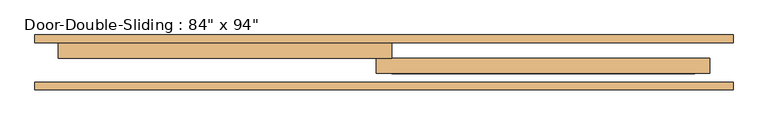
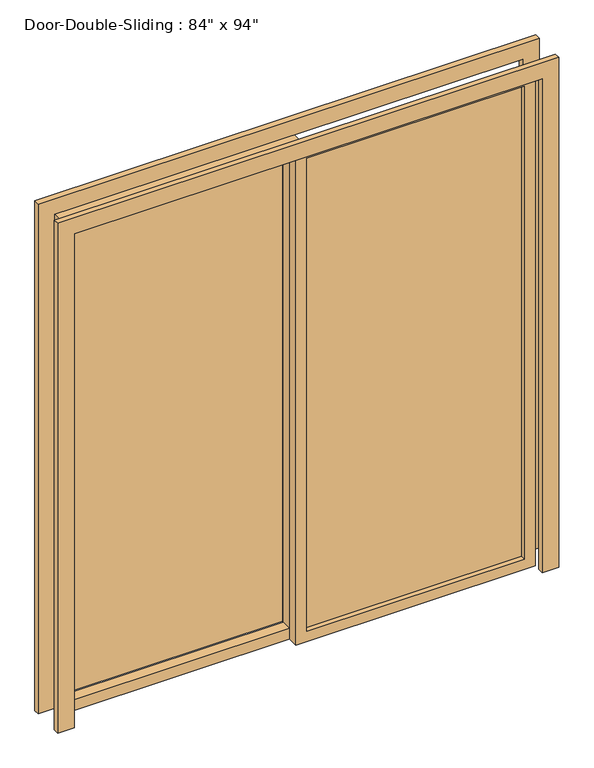
"""IFC4 building model written with IfcOpenShell, lengths in millimetres: door geometry."""

from ifc_helpers import new_model, si_unit, frame, origin, place, context, project, spatial, polyline, outline, extrude, source, transform, mapped, element, save


def door_ba072b10(model_context):
    return source(origin(), model_context, "Body", "SweptSolid", [
        extrude(outline(polyline([(0.0, 1151.2), (2476.2, 1151.2), (2476.2, -1151.2), (0.0, -1151.2), (0.0, -1075.0), (2400.0, -1075.0), (2400.0, 1075.0), (0.0, 1075.0), (0.0, 1151.2)])), frame((0.0, 192.0, 0.0), z_axis=(0.0, 1.0, 0.0), x_axis=(0.0, 0.0, 1.0)), (0.0, 0.0, 1.0), 25.4),
        extrude(outline(polyline([(0.0, -1151.2), (0.0, -1075.0), (2400.0, -1075.0), (2400.0, 1075.0), (0.0, 1075.0), (0.0, 1151.2), (2476.2, 1151.2), (2476.2, -1151.2), (0.0, -1151.2)])), frame((0.0, 36.6, 0.0), z_axis=(0.0, 1.0, 0.0), x_axis=(0.0, 0.0, 1.0)), (0.0, 0.0, 1.0), 25.4),
        extrude(outline(polyline([(2400.0, 25.4), (2400.0, -1075.0), (0.0, -1075.0), (0.0, 25.4), (2400.0, 25.4)]), holes=[polyline([(2349.2, -25.4), (50.8, -25.4), (50.8, -1024.2), (2349.2, -1024.2), (2349.2, -25.4)])]), frame((0.0, 141.2, 0.0), z_axis=(0.0, 1.0, 0.0), x_axis=(0.0, 0.0, 1.0)), (0.0, 0.0, 1.0), 50.8),
        extrude(outline(polyline([(2400.0, -25.4), (0.0, -25.4), (0.0, 1075.0), (2400.0, 1075.0), (2400.0, -25.4)]), holes=[polyline([(2349.2, 25.4), (2349.2, 1024.2), (50.8, 1024.2), (50.8, 25.4), (2349.2, 25.4)])]), frame((0.0, 90.4, 0.0), z_axis=(0.0, 1.0, 0.0), x_axis=(0.0, 0.0, 1.0)), (0.0, 0.0, 1.0), 50.8),
        extrude(outline(polyline([(-25.4, 200.025), (-1024.2, 200.025), (-1024.2, 206.375), (-25.4, 206.375), (-25.4, 200.025)])), frame((0.0, 0.0, 50.8), z_axis=(0.0, 0.0, 1.0), x_axis=(1.0, 0.0, 0.0)), (0.0, 0.0, 1.0), 2298.4),
        extrude(outline(polyline([(25.4, 118.975), (1024.2, 118.975), (1024.2, 112.625), (25.4, 112.625), (25.4, 118.975)])), frame((0.0, 0.0, 50.8), z_axis=(0.0, 0.0, 1.0), x_axis=(1.0, 0.0, 0.0)), (0.0, 0.0, 1.0), 2298.4),
    ])


if __name__ == "__main__":
    model = new_model("IFC4")
    model_context = context("Model", 3, world=origin())
    ifc_project = project(units=[si_unit("LENGTHUNIT", "METRE", prefix="MILLI")], contexts=[model_context])
    site = spatial("IfcSite", under=ifc_project)
    building = spatial("IfcBuilding", under=site)
    placement = place(None, origin())
    door_shape = door_ba072b10(model_context)
    element("IfcDoor", 1, ObjectType="Door-Double-Sliding : 84\" x 94\"", at=placement, inside=building, context=model_context, shape_type="MappedRepresentation", body=[
        mapped(door_shape, transform((0.0, 0.0, 0.0), x_axis=(1.0, 0.0, 0.0), y_axis=(0.0, 1.0, 0.0), z_axis=(0.0, 0.0, 1.0))),
    ])
    save(model, "model.ifc")

# Revit data of these elements
# Type "Door-Double-Sliding : 84\" x 94\""
#   Type Mark = "63"
#   Construction Type Id = "opn-d45"
#   Assembly Code = "C1020"
#   Analytic Construction = "Wood frame, double glass door "
#   Thickness = 50.8 mm
#   Thermal Resistance (R) = 0.31964 (m²·K)/W
#   Heat Transfer Coefficient (U) = 3.12872 W/(m²·K)
#   Height = 2400 mm
#   Rail Width = 50.8 mm
#   Stiles = 50.8 mm
#   Trim Projection Ext = 25.4 mm
#   Trim Projection Int = 25.4 mm
#   Trim Width = 76.2 mm
#   Width = 2150 mm
#   Define Thermal Properties by = 1
#   Glazing = Glass
#   Panel Material = Wood - Birch - Solid Stained Light Low Gloss
#   Trim Material = Paint - Sienna
#   Visual Light Transmittance = 0
#   Solar Heat Gain Coefficient = 0
#   Function = (empty or 0)
#   Wall Closure = (empty or 0)
# Element 1 (IfcDoor, "Door-Double-Sliding : 84\" x 94\"")
#   Materials on its faces: "Paint - Sienna", "Wood - Birch - Solid Stained Light Low Gloss", "Glass"
# Materials
#   "Glass": class "Glass", colour RGB 0 128 192, transparency 0.9, Description = "Soda Lime Glass", Cost = 0
#   "Wood - Birch - Solid Stained Light Low Gloss": class "Wood", colour RGB 210 159 95, transparency 0, Cost = 0
#   "Paint - Sienna": class "Miscellaneous", colour RGB 118 70 51, transparency 0, Cost = 0
